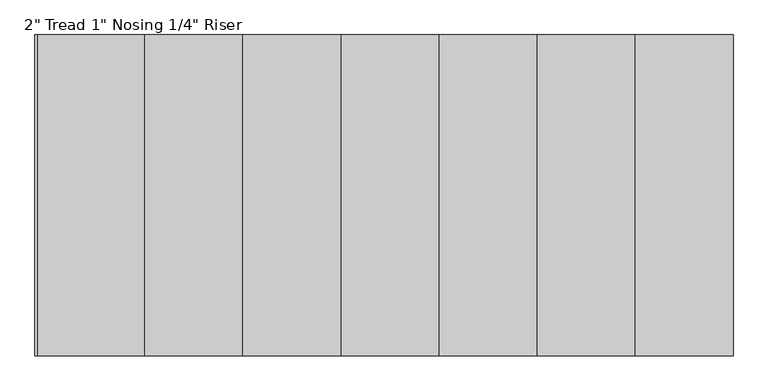
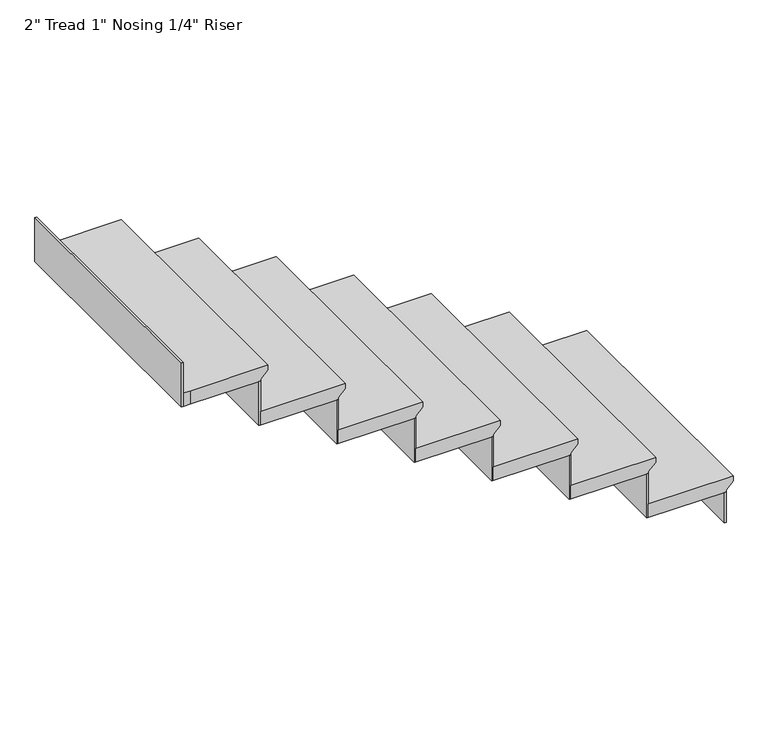
"""IFC4 building model written with IfcOpenShell, lengths in millimetres: stair flight geometry."""

from ifc_helpers import new_model, si_unit, origin, place, context, project, spatial, faceted_brep, source, transform, mapped, element, save


def stair_flight_27108a6a(model_context):
    return source(origin(), model_context, "Body", "Brep", [
        faceted_brep([(26569.9840778, 27793.0156612, 264188.575), (26569.9840778, 27793.0156612, 264207.625), (26569.9840778, 26878.6156612, 264207.625), (26569.9840778, 26878.6156612, 264188.575), (26544.5840778, 27793.0156612, 264163.175), (26544.5840778, 26878.6156612, 264163.175), (26265.1840778, 27793.0156612, 264207.625), (26265.1840778, 26878.6156612, 264207.625), (26544.5840778, 26878.6156612, 264156.825), (26265.1840778, 26878.6156612, 264156.825), (26265.1840778, 27793.0156612, 264156.825), (26544.5840778, 27793.0156612, 264156.825)], [[[0, 1, 2, 3]], [[4, 0, 3, 5]], [[2, 1, 6, 7]], [[8, 9, 10, 11]], [[2, 7, 9, 8, 5, 3]], [[8, 11, 4, 5]], [[6, 1, 0, 4, 11, 10]], [[7, 6, 10, 9]]]),
        faceted_brep([(26544.5840778, 27793.0156612, 264156.825), (26544.5840778, 27793.0156612, 264039.35), (26538.2340778, 27793.0156612, 264039.35), (26538.2340778, 27793.0156612, 264156.825), (26544.5840778, 26878.6156612, 264156.825), (26538.2340778, 26878.6156612, 264156.825), (26538.2340778, 26878.6156612, 264039.35), (26544.5840778, 26878.6156612, 264039.35)], [[[0, 1, 2, 3]], [[4, 5, 6, 7]], [[1, 0, 4, 7]], [[2, 1, 7, 6]], [[3, 2, 6, 5]], [[0, 3, 5, 4]]]),
        faceted_brep([(26265.1840778, 27793.0156612, 264325.1), (26265.1840778, 27793.0156612, 264156.825), (26258.8340778, 27793.0156612, 264156.825), (26258.8340778, 27793.0156612, 264325.1), (26265.1840778, 26878.6156612, 264325.1), (26258.8340778, 26878.6156612, 264325.1), (26258.8340778, 26878.6156612, 264156.825), (26265.1840778, 26878.6156612, 264156.825)], [[[0, 1, 2, 3]], [[4, 5, 6, 7]], [[1, 0, 4, 7]], [[2, 1, 7, 6]], [[3, 2, 6, 5]], [[0, 3, 5, 4]]]),
        faceted_brep([(26290.5840778, 26878.6156612, 264375.9), (26290.5840778, 27793.0156612, 264375.9), (25985.7840778, 27793.0156612, 264375.9), (25985.7840778, 26878.6156612, 264375.9), (26265.1840778, 26878.6156612, 264325.1), (25985.7840778, 26878.6156612, 264325.1), (25985.7840778, 27793.0156612, 264325.1), (26265.1840778, 27793.0156612, 264325.1), (26265.1840778, 26878.6156612, 264331.45), (26290.5840778, 26878.6156612, 264356.85), (26265.1840778, 27793.0156612, 264331.45), (26290.5840778, 27793.0156612, 264356.85)], [[[0, 1, 2, 3]], [[4, 5, 6, 7]], [[0, 3, 5, 4, 8, 9]], [[4, 7, 10, 8]], [[2, 1, 11, 10, 7, 6]], [[3, 2, 6, 5]], [[11, 1, 0, 9]], [[10, 11, 9, 8]]]),
        faceted_brep([(25985.7840778, 27793.0156612, 264493.375), (25985.7840778, 27793.0156612, 264325.1), (25979.4340778, 27793.0156612, 264325.1), (25979.4340778, 27793.0156612, 264493.375), (25985.7840778, 26878.6156612, 264493.375), (25979.4340778, 26878.6156612, 264493.375), (25979.4340778, 26878.6156612, 264325.1), (25985.7840778, 26878.6156612, 264325.1)], [[[0, 1, 2, 3]], [[4, 5, 6, 7]], [[1, 0, 4, 7]], [[2, 1, 7, 6]], [[3, 2, 6, 5]], [[0, 3, 5, 4]]]),
        faceted_brep([(26011.1840778, 26878.6156612, 264544.175), (26011.1840778, 27793.0156612, 264544.175), (25706.3840778, 27793.0156612, 264544.175), (25706.3840778, 26878.6156612, 264544.175), (25985.7840778, 26878.6156612, 264493.375), (25706.3840778, 26878.6156612, 264493.375), (25706.3840778, 27793.0156612, 264493.375), (25985.7840778, 27793.0156612, 264493.375), (25985.7840778, 26878.6156612, 264499.725), (26011.1840778, 26878.6156612, 264525.125), (25985.7840778, 27793.0156612, 264499.725), (26011.1840778, 27793.0156612, 264525.125)], [[[0, 1, 2, 3]], [[4, 5, 6, 7]], [[0, 3, 5, 4, 8, 9]], [[4, 7, 10, 8]], [[2, 1, 11, 10, 7, 6]], [[3, 2, 6, 5]], [[11, 1, 0, 9]], [[10, 11, 9, 8]]]),
        faceted_brep([(25706.3840778, 27793.0156612, 264661.65), (25706.3840778, 27793.0156612, 264493.375), (25700.0340778, 27793.0156612, 264493.375), (25700.0340778, 27793.0156612, 264661.65), (25706.3840778, 26878.6156612, 264661.65), (25700.0340778, 26878.6156612, 264661.65), (25700.0340778, 26878.6156612, 264493.375), (25706.3840778, 26878.6156612, 264493.375)], [[[0, 1, 2, 3]], [[4, 5, 6, 7]], [[1, 0, 4, 7]], [[2, 1, 7, 6]], [[3, 2, 6, 5]], [[0, 3, 5, 4]]]),
        faceted_brep([(25731.7840778, 26878.6156612, 264712.45), (25731.7840778, 27793.0156612, 264712.45), (25426.9840778, 27793.0156612, 264712.45), (25426.9840778, 26878.6156612, 264712.45), (25706.3840778, 26878.6156612, 264661.65), (25426.9840778, 26878.6156612, 264661.65), (25426.9840778, 27793.0156612, 264661.65), (25706.3840778, 27793.0156612, 264661.65), (25706.3840778, 26878.6156612, 264668.0), (25731.7840778, 26878.6156612, 264693.4), (25706.3840778, 27793.0156612, 264668.0), (25731.7840778, 27793.0156612, 264693.4)], [[[0, 1, 2, 3]], [[4, 5, 6, 7]], [[0, 3, 5, 4, 8, 9]], [[4, 7, 10, 8]], [[2, 1, 11, 10, 7, 6]], [[3, 2, 6, 5]], [[11, 1, 0, 9]], [[10, 11, 9, 8]]]),
        faceted_brep([(25426.9840778, 27793.0156612, 264829.925), (25426.9840778, 27793.0156612, 264661.65), (25420.6340778, 27793.0156612, 264661.65), (25420.6340778, 27793.0156612, 264829.925), (25426.9840778, 26878.6156612, 264829.925), (25420.6340778, 26878.6156612, 264829.925), (25420.6340778, 26878.6156612, 264661.65), (25426.9840778, 26878.6156612, 264661.65)], [[[0, 1, 2, 3]], [[4, 5, 6, 7]], [[1, 0, 4, 7]], [[2, 1, 7, 6]], [[3, 2, 6, 5]], [[0, 3, 5, 4]]]),
        faceted_brep([(25452.3840778, 26878.6156612, 264880.725), (25452.3840778, 27793.0156612, 264880.725), (25147.5840778, 27793.0156612, 264880.725), (25147.5840778, 26878.6156612, 264880.725), (25426.9840778, 26878.6156612, 264829.925), (25147.5840778, 26878.6156612, 264829.925), (25147.5840778, 27793.0156612, 264829.925), (25426.9840778, 27793.0156612, 264829.925), (25426.9840778, 26878.6156612, 264836.275), (25452.3840778, 26878.6156612, 264861.675), (25426.9840778, 27793.0156612, 264836.275), (25452.3840778, 27793.0156612, 264861.675)], [[[0, 1, 2, 3]], [[4, 5, 6, 7]], [[0, 3, 5, 4, 8, 9]], [[4, 7, 10, 8]], [[2, 1, 11, 10, 7, 6]], [[3, 2, 6, 5]], [[11, 1, 0, 9]], [[10, 11, 9, 8]]]),
        faceted_brep([(25147.5840778, 27793.0156612, 264998.2), (25147.5840778, 27793.0156612, 264829.925), (25141.2340778, 27793.0156612, 264829.925), (25141.2340778, 27793.0156612, 264998.2), (25147.5840778, 26878.6156612, 264998.2), (25141.2340778, 26878.6156612, 264998.2), (25141.2340778, 26878.6156612, 264829.925), (25147.5840778, 26878.6156612, 264829.925)], [[[0, 1, 2, 3]], [[4, 5, 6, 7]], [[1, 0, 4, 7]], [[2, 1, 7, 6]], [[3, 2, 6, 5]], [[0, 3, 5, 4]]]),
        faceted_brep([(25172.9840778, 26878.6156612, 265049.0), (25172.9840778, 27793.0156612, 265049.0), (24868.1840778, 27793.0156612, 265049.0), (24868.1840778, 26878.6156612, 265049.0), (25147.5840778, 26878.6156612, 264998.2), (24868.1840778, 26878.6156612, 264998.2), (24868.1840778, 27793.0156612, 264998.2), (25147.5840778, 27793.0156612, 264998.2), (25147.5840778, 26878.6156612, 265004.55), (25172.9840778, 26878.6156612, 265029.95), (25147.5840778, 27793.0156612, 265004.55), (25172.9840778, 27793.0156612, 265029.95)], [[[0, 1, 2, 3]], [[4, 5, 6, 7]], [[0, 3, 5, 4, 8, 9]], [[4, 7, 10, 8]], [[2, 1, 11, 10, 7, 6]], [[3, 2, 6, 5]], [[11, 1, 0, 9]], [[10, 11, 9, 8]]]),
        faceted_brep([(24588.7840778, 27793.0156612, 265334.75), (24588.7840778, 27793.0156612, 265166.475), (24582.4340778, 27793.0156612, 265166.475), (24582.4340778, 27793.0156612, 265334.75), (24588.7840778, 26878.6156612, 265334.75), (24582.4340778, 26878.6156612, 265334.75), (24582.4340778, 26878.6156612, 265166.475), (24588.7840778, 26878.6156612, 265166.475)], [[[0, 1, 2, 3]], [[4, 5, 6, 7]], [[1, 0, 4, 7]], [[2, 1, 7, 6]], [[3, 2, 6, 5]], [[0, 3, 5, 4]]]),
        faceted_brep([(24868.1840778, 27793.0156612, 265166.475), (24868.1840778, 27793.0156612, 264998.2), (24861.8340778, 27793.0156612, 264998.2), (24861.8340778, 27793.0156612, 265166.475), (24868.1840778, 26878.6156612, 265166.475), (24861.8340778, 26878.6156612, 265166.475), (24861.8340778, 26878.6156612, 264998.2), (24868.1840778, 26878.6156612, 264998.2)], [[[0, 1, 2, 3]], [[4, 5, 6, 7]], [[1, 0, 4, 7]], [[2, 1, 7, 6]], [[3, 2, 6, 5]], [[0, 3, 5, 4]]]),
        faceted_brep([(24588.7840778, 26878.6156612, 265217.275), (24614.1840778, 26878.6156612, 265217.275), (24893.5840778, 26878.6156612, 265217.275), (24893.5840778, 27793.0156612, 265217.275), (24614.1840778, 27793.0156612, 265217.275), (24588.7840778, 27793.0156612, 265217.275), (24614.1840778, 26878.6156612, 265166.475), (24588.7840778, 26878.6156612, 265166.475), (24588.7840778, 27793.0156612, 265166.475), (24614.1840778, 27793.0156612, 265166.475), (24868.1840778, 27793.0156612, 265166.475), (24868.1840778, 26878.6156612, 265166.475), (24868.1840778, 26878.6156612, 265172.825), (24893.5840778, 26878.6156612, 265198.225), (24868.1840778, 27793.0156612, 265172.825), (24893.5840778, 27793.0156612, 265198.225)], [[[0, 1, 2, 3, 4, 5]], [[6, 7, 8, 9, 10, 11]], [[1, 0, 7, 6]], [[2, 1, 6, 11, 12, 13]], [[11, 10, 14, 12]], [[4, 3, 15, 14, 10, 9]], [[5, 4, 9, 8]], [[0, 5, 8, 7]], [[15, 3, 2, 13]], [[14, 15, 13, 12]]]),
    ])


if __name__ == "__main__":
    model = new_model("IFC4")
    model_context = context("Model", 3, world=origin())
    ifc_project = project(units=[si_unit("LENGTHUNIT", "METRE", prefix="MILLI")], contexts=[model_context])
    site = spatial("IfcSite", under=ifc_project)
    building = spatial("IfcBuilding", under=site)
    placement = place(None, origin())
    stair_flight_shape = stair_flight_27108a6a(model_context)
    element("IfcStairFlight", 1, ObjectType="2\" Tread 1\" Nosing 1/4\" Riser", at=placement, inside=building, context=model_context, shape_type="MappedRepresentation", body=[
        mapped(stair_flight_shape, transform((0.0, 0.0, 0.0), x_axis=(1.0, 0.0, 0.0), y_axis=(0.0, 1.0, 0.0), z_axis=(0.0, 0.0, 1.0))),
    ])
    save(model, "model.ifc")

# Revit data of these elements
# Element 1 (IfcStairFlight, "2\" Tread 1\" Nosing 1/4\" Riser")
#   Materials on its faces: "SLOTTED WOOD FENCE (THERMALLY MODIFIED WOOD: ARBOR WOOD)\n(EXTERIOR STAIN : PENOFIN VERDE EXT. STAIN - COLOR: CEDAR)"
# Materials
#   "SLOTTED WOOD FENCE (THERMALLY MODIFIED WOOD: ARBOR WOOD)\n(EXTERIOR STAIN : PENOFIN VERDE EXT. STAIN - COLOR: CEDAR)": class "Wood", colour RGB 164 134 123, transparency 0, Description = "Pinus Echinata", Cost = 0
